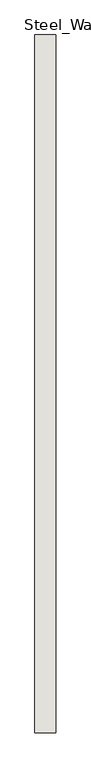
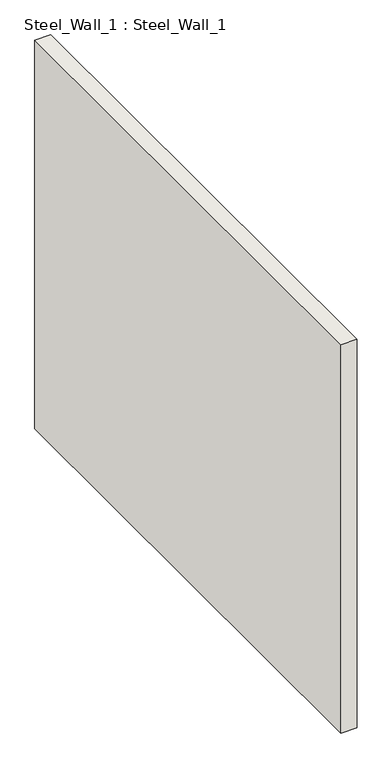
"""IFC4 building model written with IfcOpenShell, lengths in millimetres: wall geometry, Steel_Wall_1 : Steel_Wall_1."""

from ifc_helpers import new_model, si_unit, frame, origin, place, context, project, spatial, polyline, outline, extrude, source, transform, mapped, element, save


def steel_wall_1_steel_wall_1_b92ec2ca(model_context):
    return source(origin(), model_context, "Body", "SweptSolid", [
        extrude(outline(polyline([(215.0, 3755.0), (215.0, 395.0), (115.0, 395.0), (115.0, 3755.0), (215.0, 3755.0)])), frame((0.0, 0.0, 250.0), z_axis=(0.0, 0.0, 1.0), x_axis=(1.0, 0.0, 0.0)), (0.0, 0.0, 1.0), 2600.0),
    ])


if __name__ == "__main__":
    model = new_model("IFC4")
    model_context = context("Model", 3, world=origin())
    ifc_project = project(units=[si_unit("LENGTHUNIT", "METRE", prefix="MILLI")], contexts=[model_context])
    site = spatial("IfcSite", under=ifc_project)
    building = spatial("IfcBuilding", under=site)
    placement = place(None, origin())
    steel_wall_1_steel_wall_1_shape = steel_wall_1_steel_wall_1_b92ec2ca(model_context)
    element("IfcWall", 1, ObjectType="Steel_Wall_1 : Steel_Wall_1", at=placement, inside=building, context=model_context, shape_type="MappedRepresentation", body=[
        mapped(steel_wall_1_steel_wall_1_shape, transform((0.0, 0.0, 0.0), x_axis=(1.0, 0.0, 0.0), y_axis=(0.0, 1.0, 0.0), z_axis=(0.0, 0.0, 1.0))),
    ])
    save(model, "model.ifc")

# Revit data of these elements
# Type "Steel_Wall_1 : Steel_Wall_1"
#   NameOverride = "Steel_Wall_1"
# Element 1 (IfcWall, "Steel_Wall_1 : Steel_Wall_1")
#   Materials on its faces: "IfcSurfaceStyle #33"
# Materials
#   "IfcSurfaceStyle #33": class "Unassigned", colour RGB 214 214 214, transparency 0
